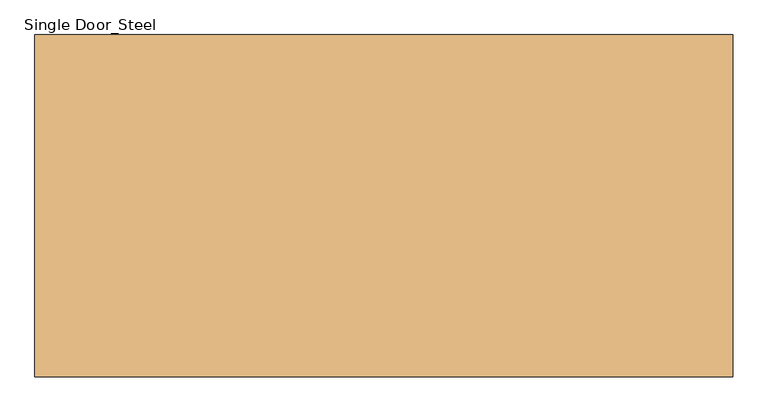
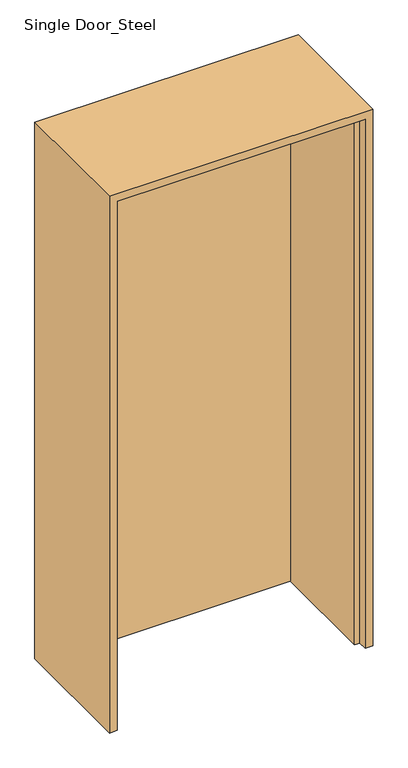
"""IFC4 building model written with IfcOpenShell, lengths in millimetres: door geometry, Single Door_Steel : H_DR_AMB_Single Door_Steel_W1000xH2150."""

import ifcopenshell
import ifcopenshell.guid

model = None  # the IFC model being written
_history = None  # IfcOwnerHistory: only IFC2X3 demands one
_inside = {}  # id of a spatial element -> (the spatial element, [elements in it])
_under = {}  # id of a project, library or spatial element -> (it, [spatial elements below it])
_declared = {}  # id of a project -> (the project, [libraries it declares])
_typed = {}  # id of a type object -> (the type object, [elements of that type])
_made_of = {}  # id of a material, layer set ... -> (it, [elements and type objects made of it])


def new_model(schema):
    """Start an empty IFC model of exactly this schema.

    Asked for "IFC4X3", IfcOpenShell would pick the latest addendum, in which some entities
    have other attributes; the version numbers below select the first issue.
    IFC2X3 requires an IfcOwnerHistory on every rooted entity: one is made here for all.
    """
    global model, _history
    if schema == "IFC4X3":
        model = ifcopenshell.file(schema_version=(4, 3, 0, 0))
    else:
        model = ifcopenshell.file(schema=schema)
    _inside.clear()
    _under.clear()
    _declared.clear()
    _typed.clear()
    _made_of.clear()
    _history = None
    if model.schema == "IFC2X3":
        org = make("IfcOrganization", Name="unknown")
        user = make(
            "IfcPersonAndOrganization",
            ThePerson=make("IfcPerson", FamilyName="unknown"),
            TheOrganization=org,
        )
        app = make(
            "IfcApplication",
            ApplicationDeveloper=org,
            Version="unknown",
            ApplicationFullName="unknown",
            ApplicationIdentifier="unknown",
        )
        _history = make(
            "IfcOwnerHistory",
            OwningUser=user,
            OwningApplication=app,
            ChangeAction="ADDED",
            CreationDate=0,
        )
    return model


def make(cls, **values):
    """One entity of the class cls with the attributes given. An attribute that is None is left unset."""
    return model.create_entity(
        cls, **{name: value for name, value in values.items() if value is not None}
    )


def rooted(cls, **values):
    """An entity with a GlobalId (a new one), such as an element, a storey or a relation."""
    return make(cls, GlobalId=ifcopenshell.guid.new(), OwnerHistory=_history, **values)


def si_unit(unit_type, name, prefix=None):
    """IfcSIUnit, for example si_unit("LENGTHUNIT", "METRE", prefix="MILLI")."""
    return make("IfcSIUnit", UnitType=unit_type, Prefix=prefix, Name=name)


def assignment(units):
    """IfcUnitAssignment: the units of a project."""
    return None if units is None else make("IfcUnitAssignment", Units=units)


def point(xyz):
    """IfcCartesianPoint."""
    return None if xyz is None else make("IfcCartesianPoint", Coordinates=xyz)


def direction(xyz):
    """IfcDirection."""
    return None if xyz is None else make("IfcDirection", DirectionRatios=xyz)


def frame(location, z_axis=None, x_axis=None):
    """IfcAxis2Placement3D, a coordinate frame: its origin and axes. An axis left out is left unset."""
    return make(
        "IfcAxis2Placement3D",
        Location=point(location),
        Axis=direction(z_axis),
        RefDirection=direction(x_axis),
    )


def origin():
    """The frame at (0, 0, 0) with its axes left unset."""
    return frame((0.0, 0.0, 0.0))


def origin_with_axes():
    """The frame at (0, 0, 0) with the z axis (0, 0, 1) and the x axis (1, 0, 0) written out."""
    return frame((0.0, 0.0, 0.0), z_axis=(0.0, 0.0, 1.0), x_axis=(1.0, 0.0, 0.0))


def place(relative_to, where):
    """IfcLocalPlacement: puts the frame where relative to a parent placement (None: the world)."""
    return make(
        "IfcLocalPlacement", PlacementRelTo=relative_to, RelativePlacement=where
    )


def context(
    kind, dimensions, precision=None, world=None, true_north=None, identifier=None
):
    """IfcGeometricRepresentationContext, for example the 3D "Model" context."""
    return make(
        "IfcGeometricRepresentationContext",
        ContextIdentifier=identifier,
        ContextType=kind,
        CoordinateSpaceDimension=dimensions,
        Precision=precision,
        WorldCoordinateSystem=world,
        TrueNorth=true_north,
    )


def project(units=None, contexts=None):
    """IfcProject with its units and contexts."""
    return rooted(
        "IfcProject",
        Name="project",
        RepresentationContexts=contexts,
        UnitsInContext=assignment(units),
    )


def spatial(cls, under=None, at=None, **own):
    """A site, building, storey or space (cls), placed at a placement, below another one or the project."""
    s = rooted(cls, ObjectPlacement=at, **own)
    if under is not None:
        _under.setdefault(under.id(), (under, []))[1].append(s)
    return s


def polyline(points):
    """IfcPolyline through the points."""
    return make("IfcPolyline", Points=[point(p) for p in points])


def outline(outer, holes=None, kind="AREA"):
    """IfcArbitraryClosedProfileDef: a profile drawn as a closed curve; with holes, ...WithVoids."""
    if holes is None:
        return make("IfcArbitraryClosedProfileDef", ProfileType=kind, OuterCurve=outer)
    return make(
        "IfcArbitraryProfileDefWithVoids",
        ProfileType=kind,
        OuterCurve=outer,
        InnerCurves=holes,
    )


def extrude(swept, where, along, depth):
    """IfcExtrudedAreaSolid: the profile swept, set in the frame where, extruded along a direction by depth."""
    return make(
        "IfcExtrudedAreaSolid",
        SweptArea=swept,
        Position=where,
        ExtrudedDirection=direction(along),
        Depth=depth,
    )


def faces_of(points, faces, orient=None, outer=None):
    """IfcFace entities. A face is a list of loops; a loop is a list of indices into points, from 0.

    orient and outer hold one flag for each loop. By default every Orientation is true, the
    first loop of a face is its IfcFaceOuterBound and the others are IfcFaceBound.
    """
    made = []
    for i, loops in enumerate(faces):
        bounds = []
        for j, loop in enumerate(loops):
            is_outer = j == 0 if outer is None else outer[i][j]
            bounds.append(
                make(
                    "IfcFaceOuterBound" if is_outer else "IfcFaceBound",
                    Bound=make("IfcPolyLoop", Polygon=[points[k] for k in loop]),
                    Orientation=True if orient is None else orient[i][j],
                )
            )
        made.append(make("IfcFace", Bounds=bounds))
    return made


def faceted_brep(points, faces, orient=None, outer=None, voids=None):
    """IfcFacetedBrep: a solid bounded by flat faces; with voids (closed shells), ...WithVoids."""
    shared = [point(p) for p in points]
    hull = make("IfcClosedShell", CfsFaces=faces_of(shared, faces, orient, outer))
    if voids is None:
        return make("IfcFacetedBrep", Outer=hull)
    return make(
        "IfcFacetedBrepWithVoids",
        Outer=hull,
        Voids=[
            make(cls, CfsFaces=faces_of(shared, fs, o, b)) for cls, fs, o, b in voids
        ],
    )


def shape(context_of_items, identifier, shape_type, items):
    """IfcShapeRepresentation: the items that make up one representation, for example the "Body"."""
    return make(
        "IfcShapeRepresentation",
        ContextOfItems=context_of_items,
        RepresentationIdentifier=identifier,
        RepresentationType=shape_type,
        Items=items,
    )


def source(mapping_origin, context_of_items, identifier, shape_type, items):
    """IfcRepresentationMap: a shape defined once, which mapped items show again and again."""
    return make(
        "IfcRepresentationMap",
        MappingOrigin=mapping_origin,
        MappedRepresentation=shape(context_of_items, identifier, shape_type, items),
    )


def transform(
    local_origin,
    x_axis=None,
    y_axis=None,
    z_axis=None,
    scale=None,
    scale2=None,
    scale3=None,
    uniform=True,
):
    """IfcCartesianTransformationOperator3D, or its non-uniform kind. x_axis, y_axis, z_axis: its Axis1, 2, 3."""
    if uniform:
        return make(
            "IfcCartesianTransformationOperator3D",
            Axis1=direction(x_axis),
            Axis2=direction(y_axis),
            LocalOrigin=point(local_origin),
            Scale=scale,
            Axis3=direction(z_axis),
        )
    return make(
        "IfcCartesianTransformationOperator3DnonUniform",
        Axis1=direction(x_axis),
        Axis2=direction(y_axis),
        LocalOrigin=point(local_origin),
        Scale=scale,
        Axis3=direction(z_axis),
        Scale2=scale2,
        Scale3=scale3,
    )


def mapped(mapping_source, mapping_target):
    """IfcMappedItem: shows the shape of a source again, moved by a transform."""
    return make(
        "IfcMappedItem", MappingSource=mapping_source, MappingTarget=mapping_target
    )


def made_of(thing, what):
    """Note that an element or type object is made of a material, layer set ...; save() writes the relation."""
    if what is not None:
        _made_of.setdefault(what.id(), (what, []))[1].append(thing)
    return thing


def element(
    cls,
    number,
    at=None,
    inside=None,
    cuts=None,
    type_object=None,
    material=None,
    context=None,
    identifier="Body",
    shape_type=None,
    held_by="IfcProductDefinitionShape",
    body=None,
    shapes=None,
    **own,
):
    """One element of the class cls, such as IfcWall. Its Tag is "e" and its number.

    at: its placement. inside: the storey or other place that contains it. cuts: it is an
    opening in that element (IfcRelVoidsElement). A single representation is given by context,
    identifier, shape_type and body (its items); several are given by shapes. held_by: the class
    of the entity that holds the representations. save() writes the other relations.
    """
    e = rooted(cls, Tag="e%d" % number, ObjectPlacement=at, **own)
    if body is not None:
        shapes = [shape(context, identifier, shape_type, body)]
    if shapes is not None:
        e.Representation = make(held_by, Representations=shapes)
    if inside is not None:
        _inside.setdefault(inside.id(), (inside, []))[1].append(e)
    if cuts is not None:
        rooted(
            "IfcRelVoidsElement", RelatingBuildingElement=cuts, RelatedOpeningElement=e
        )
    if type_object is not None:
        _typed.setdefault(type_object.id(), (type_object, []))[1].append(e)
    return made_of(e, material)


def aggregate(whole, parts):
    """IfcRelAggregates: a whole, such as a stair, and the parts it consists of."""
    return rooted("IfcRelAggregates", RelatingObject=whole, RelatedObjects=parts)


def save(model, path):
    """Write the relations noted so far, then the file.

    IfcRelAggregates (storeys below a building ...), IfcRelContainedInSpatialStructure (elements
    in a storey), IfcRelDefinesByType, IfcRelAssociatesMaterial and IfcRelDeclares: one each for
    every whole, place, type object, material and project.
    """
    for whole, parts in _under.values():
        aggregate(whole, parts)
    for where, things in _inside.values():
        rooted(
            "IfcRelContainedInSpatialStructure",
            RelatedElements=things,
            RelatingStructure=where,
        )
    for kind, things in _typed.values():
        rooted("IfcRelDefinesByType", RelatedObjects=things, RelatingType=kind)
    for what, things in _made_of.values():
        rooted("IfcRelAssociatesMaterial", RelatedObjects=things, RelatingMaterial=what)
    for by, libraries in _declared.values():
        rooted("IfcRelDeclares", RelatingContext=by, RelatedDefinitions=libraries)
    model.write(path)


def single_door_steel_7afc0ab2(model_context):
    return source(origin(), model_context, "Body", "SolidModel", [
        extrude(outline(polyline([(470.0, 245.0), (470.0, 210.0), (-470.0, 210.0), (-470.0, 245.0), (470.0, 245.0)])), origin_with_axes(), (0.0, 0.0, 1.0), 2120.0),
        faceted_brep([(470.0, 245.0, 0.0), (500.0, 245.0, 0.0), (500.0, -245.0, 0.0), (470.0, -245.0, 0.0), (470.0, -210.0, 0.0), (450.0, -210.0, 0.0), (450.0, 210.0, 0.0), (470.0, 210.0, 0.0), (470.0, 245.0, 2120.0), (-470.0, 245.0, 2120.0), (-470.0, 245.0, 0.0), (-500.0, 245.0, 0.0), (-500.0, 245.0, 2150.0), (500.0, 245.0, 2150.0), (500.0, -245.0, 2150.0), (-500.0, -245.0, 2150.0), (-500.0, -245.0, 0.0), (-470.0, -245.0, 0.0), (-470.0, -245.0, 2120.0), (470.0, -245.0, 2120.0), (470.0, -210.0, 2120.0), (-470.0, -210.0, 2120.0), (-470.0, -210.0, 0.0), (-450.0, -210.0, 0.0), (-450.0, -210.0, 2100.0), (450.0, -210.0, 2100.0), (450.0, 210.0, 2100.0), (-450.0, 210.0, 2100.0), (-450.0, 210.0, 0.0), (-470.0, 210.0, 0.0), (-470.0, 210.0, 2120.0), (470.0, 210.0, 2120.0)], [[[0, 1, 2, 3, 4, 5, 6, 7]], [[1, 0, 8, 9, 10, 11, 12, 13]], [[2, 1, 13, 14]], [[3, 2, 14, 15, 16, 17, 18, 19]], [[4, 3, 19, 20]], [[5, 4, 20, 21, 22, 23, 24, 25]], [[6, 5, 25, 26]], [[7, 6, 26, 27, 28, 29, 30, 31]], [[0, 7, 31, 8]], [[9, 30, 29, 10]], [[10, 29, 28, 23, 22, 17, 16, 11]], [[15, 12, 11, 16]], [[21, 18, 17, 22]], [[27, 24, 23, 28]], [[14, 13, 12, 15]], [[20, 19, 18, 21]], [[26, 25, 24, 27]], [[8, 31, 30, 9]]]),
    ])


if __name__ == "__main__":
    model = new_model("IFC4")
    model_context = context("Model", 3, world=origin())
    ifc_project = project(units=[si_unit("LENGTHUNIT", "METRE", prefix="MILLI")], contexts=[model_context])
    site = spatial("IfcSite", under=ifc_project)
    building = spatial("IfcBuilding", under=site)
    placement = place(None, origin())
    single_door_steel_shape = single_door_steel_7afc0ab2(model_context)
    element("IfcDoor", 1, ObjectType="Single Door_Steel : H_DR_AMB_Single Door_Steel_W1000xH2150", at=placement, inside=building, context=model_context, shape_type="MappedRepresentation", body=[
        mapped(single_door_steel_shape, transform((0.0, 0.0, 0.0), x_axis=(1.0, 0.0, 0.0), y_axis=(0.0, 1.0, 0.0), z_axis=(0.0, 0.0, 1.0))),
    ])
    save(model, "model.ifc")

# Revit data of these elements
# Type "Single Door_Steel : H_DR_AMB_Single Door_Steel_W1000xH2150"
#   Type Mark = "364"
#   Analytic Construction = "<None>"
#   프레임 투영 외부. = 25.000 mm
#   프레임 투영 내부. = 25.000 mm
#   프레임 폭 = 75.000 mm
#   Height = 2150.000 mm
#   Width = 1000.000 mm
#   Define Thermal Properties by = 1
#   문 패널 = none
#   문 프레임 = none
#   Function = (empty or 0)
#   Wall Closure = (empty or 0)
